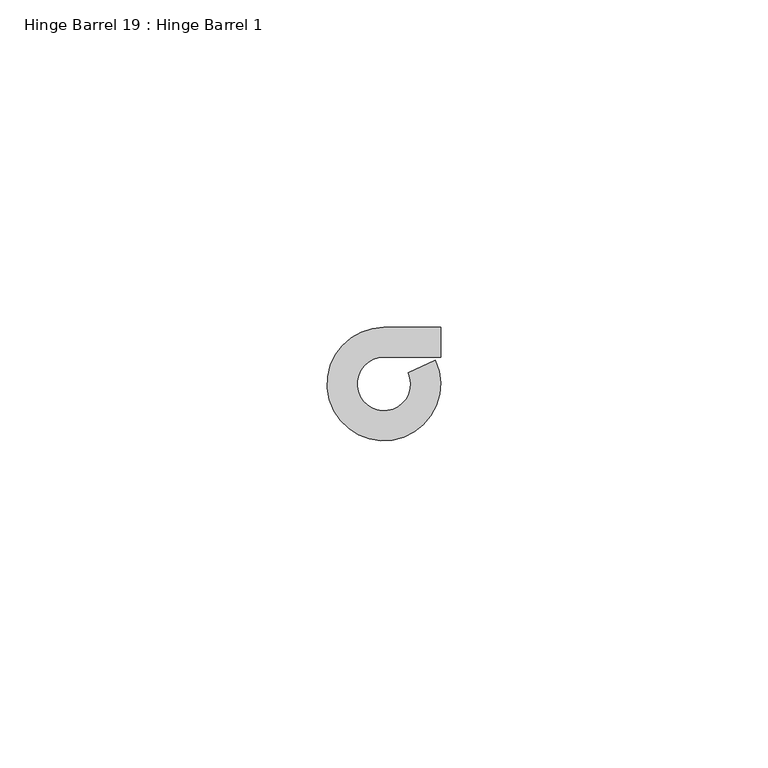
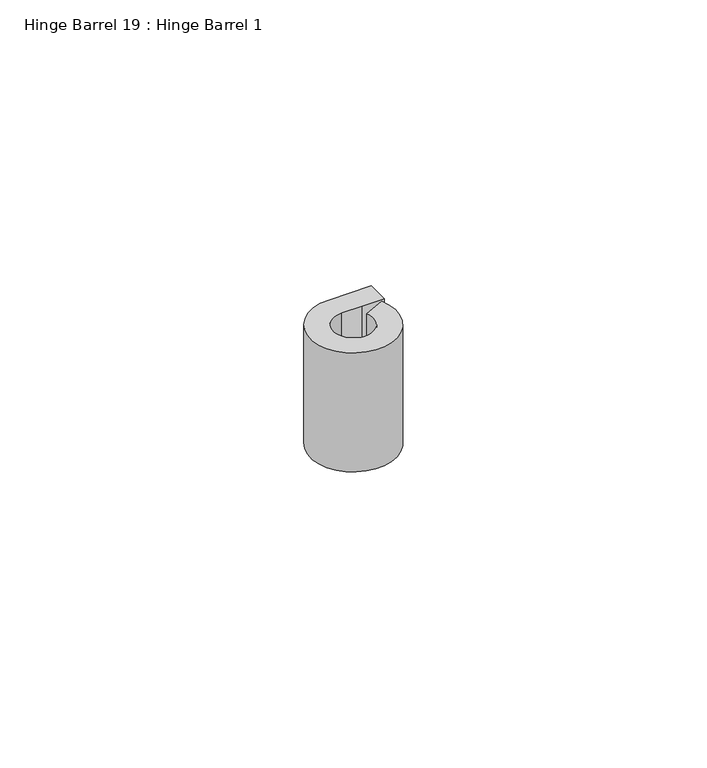
"""IFC4 building model written with IfcOpenShell, lengths in millimetres: proxy geometry, Hinge Barrel 19 : Hinge Barrel 1."""

from ifc_helpers import new_model, si_unit, point, frame, frame_2d, origin, place, context, project, spatial, polyline, circle_curve, trimmed, segment, composite_curve, outline, extrude, source, transform, mapped, element, save


def hinge_barrel_19_hinge_barrel_1_935fc850(model_context):
    return source(origin(), model_context, "Body", "SweptSolid", [
        extrude(outline(composite_curve([segment(polyline([(587323.2214739, -533980.5883841), (587319.1320739, -533980.5883841)]), True, "CONTINUOUS"), segment(trimmed(circle_curve(frame_2d((587319.1320739, -533984.6777841)), 4.0894), [point((587319.1320739, -533980.5883841))], [point((587322.8436736, -533982.9610371))], True, "CARTESIAN"), True, "CONTINUOUS"), segment(polyline([(587322.8436736, -533982.9610371), (587326.986084, -533981.0450249)]), True, "CONTINUOUS"), segment(trimmed(circle_curve(frame_2d((587319.1320739, -533984.6777841)), 8.6534625), [point((587326.986084, -533981.0450249))], [point((587319.1320739, -533976.0243216))], False, "CARTESIAN"), True, "CONTINUOUS"), segment(polyline([(587319.1320739, -533976.0243216), (587327.7934739, -533976.0243216), (587327.7934739, -533980.5883841), (587323.2214739, -533980.5883841)]), True, "CONTINUOUS")], self_intersect=False)), frame((0.0, 0.0, 1936.75), z_axis=(0.0, 0.0, 1.0), x_axis=(1.0, 0.0, 0.0)), (0.0, 0.0, 1.0), 25.4),
    ])


if __name__ == "__main__":
    model = new_model("IFC4")
    model_context = context("Model", 3, world=origin())
    ifc_project = project(units=[si_unit("LENGTHUNIT", "METRE", prefix="MILLI")], contexts=[model_context])
    site = spatial("IfcSite", under=ifc_project)
    building = spatial("IfcBuilding", under=site)
    placement = place(None, origin())
    hinge_barrel_19_hinge_barrel_1_shape = hinge_barrel_19_hinge_barrel_1_935fc850(model_context)
    element("IfcBuildingElementProxy", 1, Name="Hinge Barrel 19 : Hinge Barrel 1", ObjectType="Hinge Barrel 19 : Hinge Barrel 1", at=placement, inside=building, context=model_context, shape_type="MappedRepresentation", body=[
        mapped(hinge_barrel_19_hinge_barrel_1_shape, transform((0.0, 0.0, 0.0), x_axis=(1.0, 0.0, 0.0), y_axis=(0.0, 1.0, 0.0), z_axis=(0.0, 0.0, 1.0))),
    ])
    save(model, "model.ifc")

# Revit data of these elements
# Element 1 (IfcBuildingElementProxy, "Hinge Barrel 19 : Hinge Barrel 1")
#   Materials on its faces: "6\"X6\" WELD-ON STL BUTT HINGE"
# Materials
#   "6\"X6\" WELD-ON STL BUTT HINGE": class "Metal", colour RGB 189 187 185, transparency 0, Description = "Carbon steel", Cost = 0
